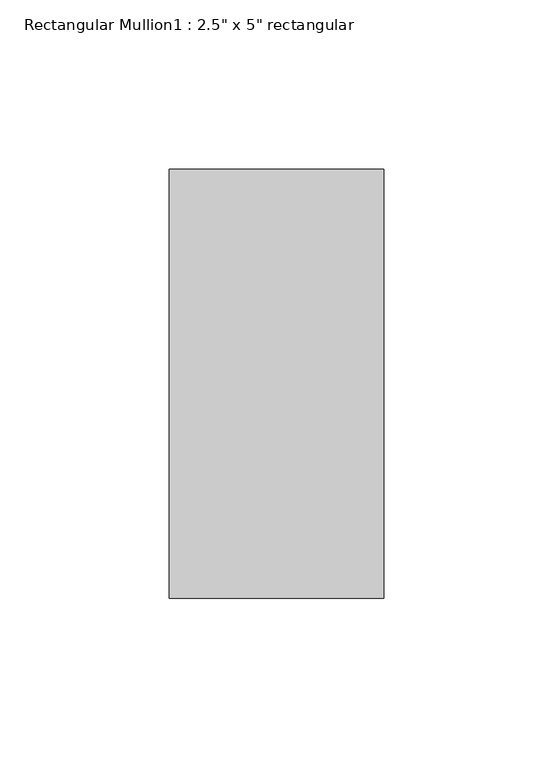
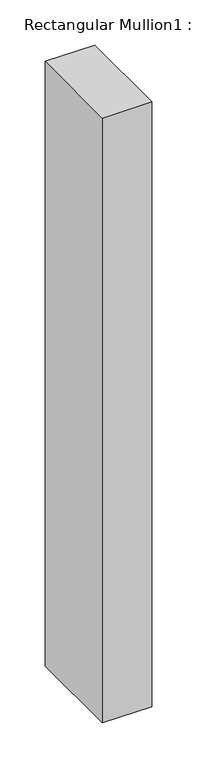
"""IFC4 building model written with IfcOpenShell, lengths in millimetres: member geometry."""

from ifc_helpers import new_model, si_unit, frame, origin, place, context, project, spatial, polyline, outline, extrude, source, transform, mapped, element, save


def member_ad567e07(model_context):
    return source(origin(), model_context, "Body", "SweptSolid", [
        extrude(outline(polyline([(31.75, 63.5), (31.75, -63.5), (-31.75, -63.5), (-31.75, 63.5), (31.75, 63.5)])), frame((0.0, 0.0, -819.15), z_axis=(0.0, 0.0, 1.0), x_axis=(1.0, 0.0, 0.0)), (0.0, 0.0, 1.0), 819.15),
    ])


if __name__ == "__main__":
    model = new_model("IFC4")
    model_context = context("Model", 3, world=origin())
    ifc_project = project(units=[si_unit("LENGTHUNIT", "METRE", prefix="MILLI")], contexts=[model_context])
    site = spatial("IfcSite", under=ifc_project)
    building = spatial("IfcBuilding", under=site)
    placement = place(None, origin())
    member_shape = member_ad567e07(model_context)
    element("IfcMember", 1, ObjectType="Rectangular Mullion1 : 2.5\" x 5\" rectangular", at=placement, inside=building, context=model_context, shape_type="MappedRepresentation", body=[
        mapped(member_shape, transform((0.0, 0.0, 0.0), x_axis=(1.0, 0.0, 0.0), y_axis=(0.0, 1.0, 0.0), z_axis=(0.0, 0.0, 1.0))),
    ])
    save(model, "model.ifc")

# Revit data of these elements
# Type "Rectangular Mullion1 : 2.5\" x 5\" rectangular"
#   built-in parameter 1007304 = 0.416667 (stored number, unit not read)
#   built-in parameter 1007301 = 0.104167 (stored number, unit not read)
#   built-in parameter 1007300 = 0.104167 (stored number, unit not read)
# Element 1 (IfcMember, "Rectangular Mullion1 : 2.5\" x 5\" rectangular")
#   Materials on its faces: "support-frame"
# Materials
#   "support-frame": class "Unassigned", colour RGB 233 233 233, transparency 0, Cost = 0
